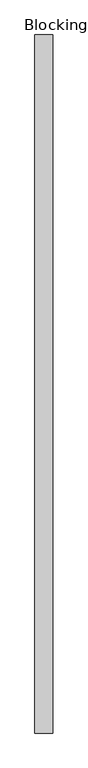
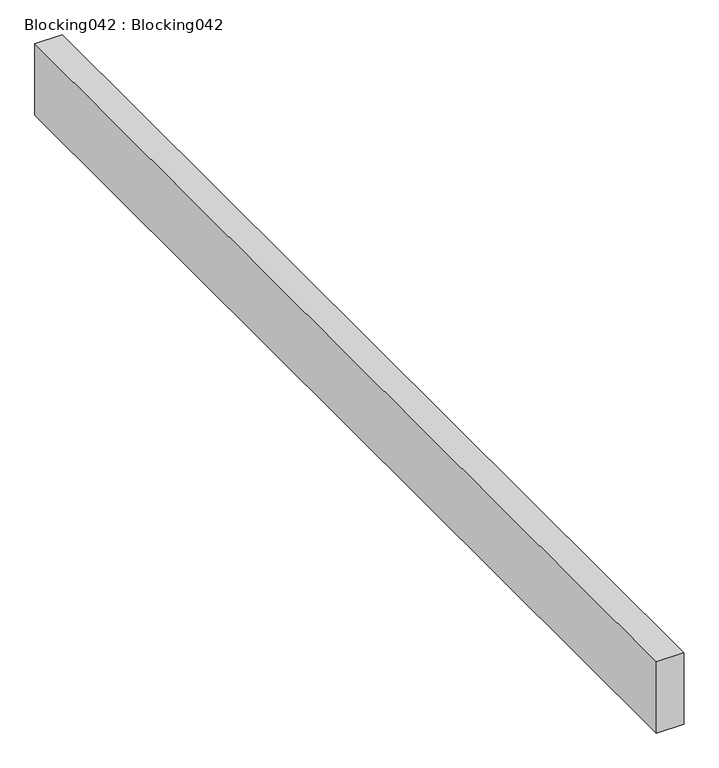
"""IFC4 building model written with IfcOpenShell, lengths in millimetres: proxy geometry, Blocking042 : Blocking042."""

from ifc_helpers import new_model, si_unit, frame, origin, place, context, project, spatial, polyline, outline, extrude, source, transform, mapped, element, save


def blocking042_blocking042_94a626ea(model_context):
    return source(origin(), model_context, "Body", "SweptSolid", [
        extrude(outline(polyline([(-4423.2538825, -1052.8908936), (-4474.0538825, -1052.8908936), (-4474.0538825, 947.1091064), (-4423.2538825, 947.1091064), (-4423.2538825, -1052.8908936)])), frame((0.0, 0.0, 39579.2960083), z_axis=(0.0, 0.0, 1.0), x_axis=(1.0, 0.0, 0.0)), (0.0, 0.0, 1.0), 139.7),
    ])


if __name__ == "__main__":
    model = new_model("IFC4")
    model_context = context("Model", 3, world=origin())
    ifc_project = project(units=[si_unit("LENGTHUNIT", "METRE", prefix="MILLI")], contexts=[model_context])
    site = spatial("IfcSite", under=ifc_project)
    building = spatial("IfcBuilding", under=site)
    placement = place(None, origin())
    blocking042_blocking042_shape = blocking042_blocking042_94a626ea(model_context)
    element("IfcBuildingElementProxy", 1, Name="Blocking042 : Blocking042", ObjectType="Blocking042 : Blocking042", at=placement, inside=building, context=model_context, shape_type="MappedRepresentation", body=[
        mapped(blocking042_blocking042_shape, transform((0.0, 0.0, 0.0), x_axis=(1.0, 0.0, 0.0), y_axis=(0.0, 1.0, 0.0), z_axis=(0.0, 0.0, 1.0))),
    ])
    save(model, "model.ifc")

# Revit data of these elements
# Type "Blocking042 : Blocking042"
#   NameOverride = "Blocking042"
# Element 1 (IfcBuildingElementProxy, "Blocking042 : Blocking042")
#   Materials on its faces: "WOOD BLOCKING AS REQUIRED"
# Materials
#   "WOOD BLOCKING AS REQUIRED": class "Unassigned", colour RGB 166 124 85, transparency 0, Cost = 0
